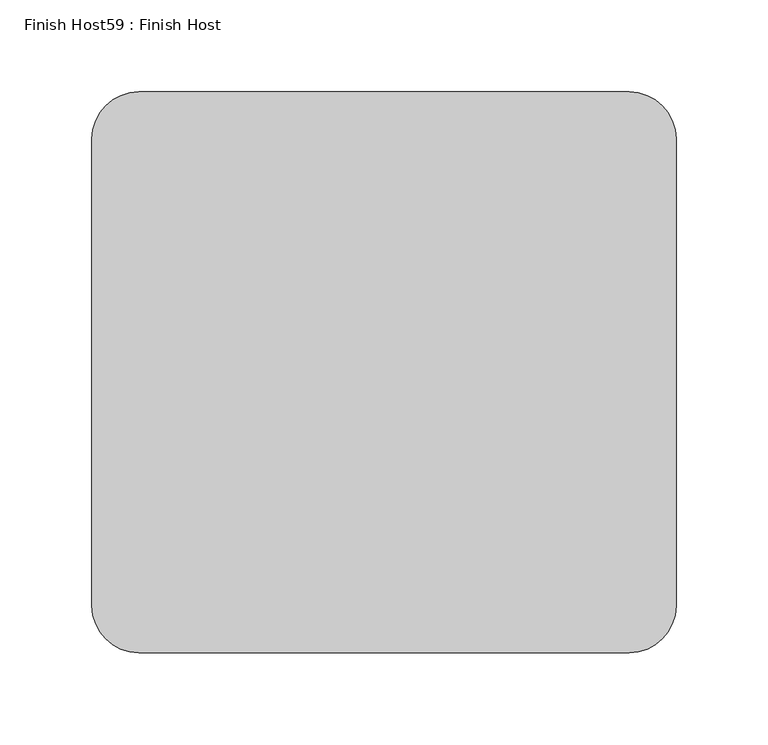
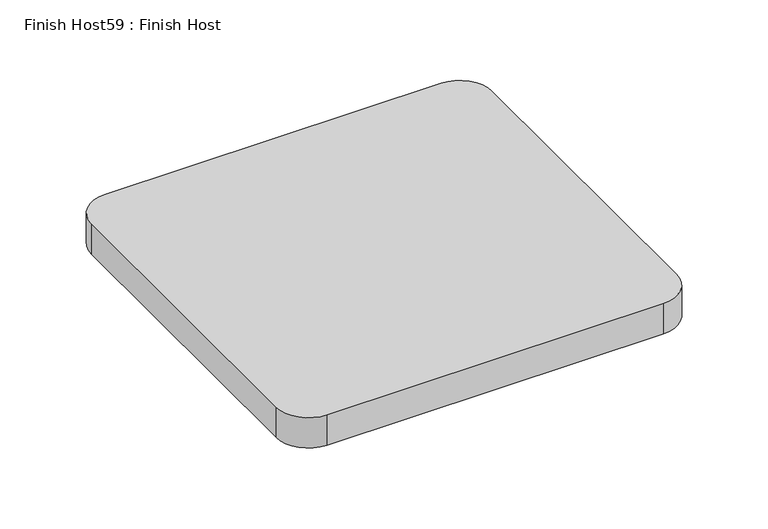
"""IFC4 building model written with IfcOpenShell, lengths in millimetres: proxy geometry, Finish Host59 : Finish Host."""

from ifc_helpers import new_model, si_unit, point, frame_2d, origin, origin_with_axes, place, context, project, spatial, polyline, circle_curve, trimmed, segment, composite_curve, outline, extrude, source, transform, mapped, element, save


def finish_host59_finish_host_a72447a2(model_context):
    return source(origin(), model_context, "Body", "SweptSolid", [
        extrude(outline(composite_curve([segment(polyline([(-16287.7939795, 12994.4419385), (-16287.7939795, 13248.4419385)]), True, "CONTINUOUS"), segment(trimmed(circle_curve(frame_2d((-16262.3939795, 13248.4419385)), 25.4), [point((-16287.7939795, 13248.4419385))], [point((-16262.3939795, 13273.8419385))], False, "CARTESIAN"), True, "CONTINUOUS"), segment(polyline([(-16262.3939795, 13273.8419385), (-15995.6939795, 13273.8419385)]), True, "CONTINUOUS"), segment(trimmed(circle_curve(frame_2d((-15995.6939795, 13248.4419385)), 25.4), [point((-15995.6939795, 13273.8419385))], [point((-15970.2939795, 13248.4419385))], False, "CARTESIAN"), True, "CONTINUOUS"), segment(polyline([(-15970.2939795, 13248.4419385), (-15970.2939795, 12994.4419385)]), True, "CONTINUOUS"), segment(trimmed(circle_curve(frame_2d((-15995.6939795, 12994.4419385)), 25.4), [point((-15970.2939795, 12994.4419385))], [point((-15995.6939795, 12969.0419385))], False, "CARTESIAN"), True, "CONTINUOUS"), segment(polyline([(-15995.6939795, 12969.0419385), (-16262.3939795, 12969.0419385)]), True, "CONTINUOUS"), segment(trimmed(circle_curve(frame_2d((-16262.3939795, 12994.4419385)), 25.4), [point((-16262.3939795, 12969.0419385))], [point((-16287.7939795, 12994.4419385))], False, "CARTESIAN"), True, "CONTINUOUS")], self_intersect=False)), origin_with_axes(), (0.0, 0.0, 1.0), 25.4),
    ])


if __name__ == "__main__":
    model = new_model("IFC4")
    model_context = context("Model", 3, world=origin())
    ifc_project = project(units=[si_unit("LENGTHUNIT", "METRE", prefix="MILLI")], contexts=[model_context])
    site = spatial("IfcSite", under=ifc_project)
    building = spatial("IfcBuilding", under=site)
    placement = place(None, origin())
    finish_host59_finish_host_shape = finish_host59_finish_host_a72447a2(model_context)
    element("IfcBuildingElementProxy", 1, Name="Finish Host59 : Finish Host", ObjectType="Finish Host59 : Finish Host", at=placement, inside=building, context=model_context, shape_type="MappedRepresentation", body=[
        mapped(finish_host59_finish_host_shape, transform((0.0, 0.0, 0.0), x_axis=(1.0, 0.0, 0.0), y_axis=(0.0, 1.0, 0.0), z_axis=(0.0, 0.0, 1.0))),
    ])
    save(model, "model.ifc")

# Revit data of these elements
# Type "Finish Host59 : Finish Host"
#   Countertop Material = none
# Element 1 (IfcBuildingElementProxy, "Finish Host59 : Finish Host")
#   Materials on its faces: "Thread - Teknion - Golden Brown"
# Materials
#   "Thread - Teknion - Golden Brown": class "Fabric", colour RGB 134 101 60, transparency 0, Model = "F206", Manufacturer = "Teknion Studio", URL = "http://www.teknion.com/", Description = "Fantasme Full Wool", Cost = 0
